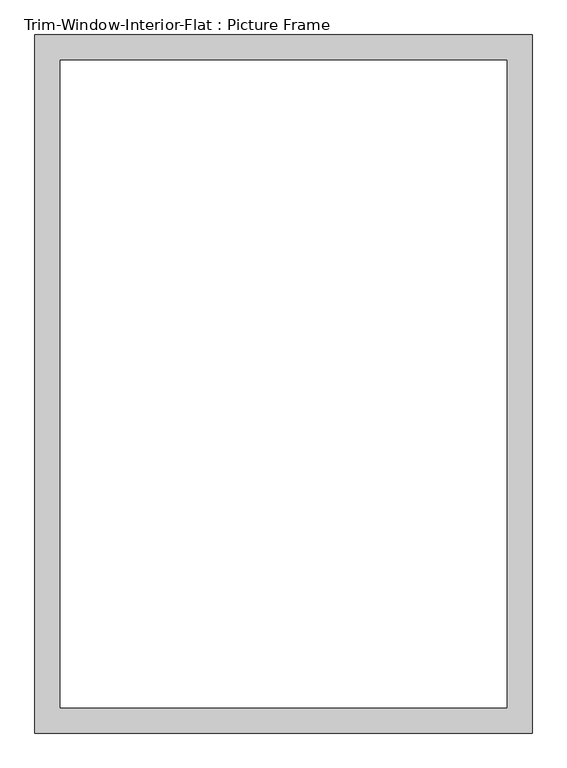
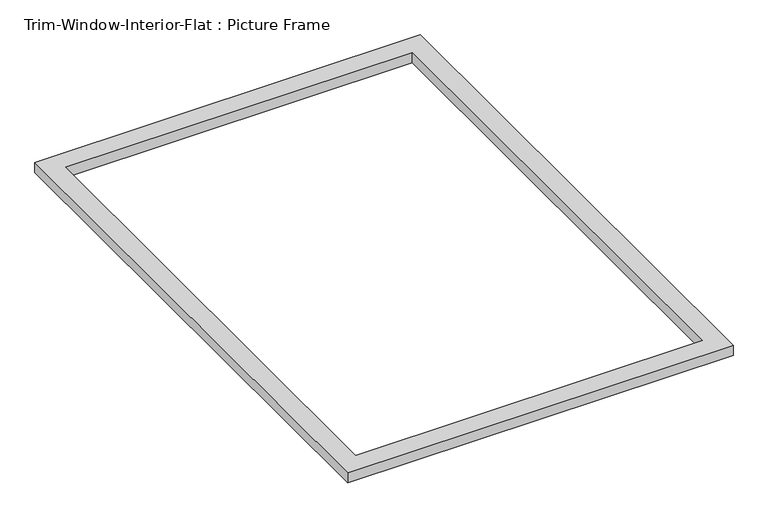
"""IFC4 building model written with IfcOpenShell, lengths in millimetres: proxy geometry, Trim-Window-Interior-Flat : Picture Frame."""

import ifcopenshell
import ifcopenshell.guid

model = None  # the IFC model being written
_history = None  # IfcOwnerHistory: only IFC2X3 demands one
_inside = {}  # id of a spatial element -> (the spatial element, [elements in it])
_under = {}  # id of a project, library or spatial element -> (it, [spatial elements below it])
_declared = {}  # id of a project -> (the project, [libraries it declares])
_typed = {}  # id of a type object -> (the type object, [elements of that type])
_made_of = {}  # id of a material, layer set ... -> (it, [elements and type objects made of it])


def new_model(schema):
    """Start an empty IFC model of exactly this schema.

    Asked for "IFC4X3", IfcOpenShell would pick the latest addendum, in which some entities
    have other attributes; the version numbers below select the first issue.
    IFC2X3 requires an IfcOwnerHistory on every rooted entity: one is made here for all.
    """
    global model, _history
    if schema == "IFC4X3":
        model = ifcopenshell.file(schema_version=(4, 3, 0, 0))
    else:
        model = ifcopenshell.file(schema=schema)
    _inside.clear()
    _under.clear()
    _declared.clear()
    _typed.clear()
    _made_of.clear()
    _history = None
    if model.schema == "IFC2X3":
        org = make("IfcOrganization", Name="unknown")
        user = make(
            "IfcPersonAndOrganization",
            ThePerson=make("IfcPerson", FamilyName="unknown"),
            TheOrganization=org,
        )
        app = make(
            "IfcApplication",
            ApplicationDeveloper=org,
            Version="unknown",
            ApplicationFullName="unknown",
            ApplicationIdentifier="unknown",
        )
        _history = make(
            "IfcOwnerHistory",
            OwningUser=user,
            OwningApplication=app,
            ChangeAction="ADDED",
            CreationDate=0,
        )
    return model


def make(cls, **values):
    """One entity of the class cls with the attributes given. An attribute that is None is left unset."""
    return model.create_entity(
        cls, **{name: value for name, value in values.items() if value is not None}
    )


def rooted(cls, **values):
    """An entity with a GlobalId (a new one), such as an element, a storey or a relation."""
    return make(cls, GlobalId=ifcopenshell.guid.new(), OwnerHistory=_history, **values)


def si_unit(unit_type, name, prefix=None):
    """IfcSIUnit, for example si_unit("LENGTHUNIT", "METRE", prefix="MILLI")."""
    return make("IfcSIUnit", UnitType=unit_type, Prefix=prefix, Name=name)


def assignment(units):
    """IfcUnitAssignment: the units of a project."""
    return None if units is None else make("IfcUnitAssignment", Units=units)


def point(xyz):
    """IfcCartesianPoint."""
    return None if xyz is None else make("IfcCartesianPoint", Coordinates=xyz)


def direction(xyz):
    """IfcDirection."""
    return None if xyz is None else make("IfcDirection", DirectionRatios=xyz)


def frame(location, z_axis=None, x_axis=None):
    """IfcAxis2Placement3D, a coordinate frame: its origin and axes. An axis left out is left unset."""
    return make(
        "IfcAxis2Placement3D",
        Location=point(location),
        Axis=direction(z_axis),
        RefDirection=direction(x_axis),
    )


def origin():
    """The frame at (0, 0, 0) with its axes left unset."""
    return frame((0.0, 0.0, 0.0))


def origin_with_axes():
    """The frame at (0, 0, 0) with the z axis (0, 0, 1) and the x axis (1, 0, 0) written out."""
    return frame((0.0, 0.0, 0.0), z_axis=(0.0, 0.0, 1.0), x_axis=(1.0, 0.0, 0.0))


def place(relative_to, where):
    """IfcLocalPlacement: puts the frame where relative to a parent placement (None: the world)."""
    return make(
        "IfcLocalPlacement", PlacementRelTo=relative_to, RelativePlacement=where
    )


def context(
    kind, dimensions, precision=None, world=None, true_north=None, identifier=None
):
    """IfcGeometricRepresentationContext, for example the 3D "Model" context."""
    return make(
        "IfcGeometricRepresentationContext",
        ContextIdentifier=identifier,
        ContextType=kind,
        CoordinateSpaceDimension=dimensions,
        Precision=precision,
        WorldCoordinateSystem=world,
        TrueNorth=true_north,
    )


def project(units=None, contexts=None):
    """IfcProject with its units and contexts."""
    return rooted(
        "IfcProject",
        Name="project",
        RepresentationContexts=contexts,
        UnitsInContext=assignment(units),
    )


def spatial(cls, under=None, at=None, **own):
    """A site, building, storey or space (cls), placed at a placement, below another one or the project."""
    s = rooted(cls, ObjectPlacement=at, **own)
    if under is not None:
        _under.setdefault(under.id(), (under, []))[1].append(s)
    return s


def polyline(points):
    """IfcPolyline through the points."""
    return make("IfcPolyline", Points=[point(p) for p in points])


def outline(outer, holes=None, kind="AREA"):
    """IfcArbitraryClosedProfileDef: a profile drawn as a closed curve; with holes, ...WithVoids."""
    if holes is None:
        return make("IfcArbitraryClosedProfileDef", ProfileType=kind, OuterCurve=outer)
    return make(
        "IfcArbitraryProfileDefWithVoids",
        ProfileType=kind,
        OuterCurve=outer,
        InnerCurves=holes,
    )


def extrude(swept, where, along, depth):
    """IfcExtrudedAreaSolid: the profile swept, set in the frame where, extruded along a direction by depth."""
    return make(
        "IfcExtrudedAreaSolid",
        SweptArea=swept,
        Position=where,
        ExtrudedDirection=direction(along),
        Depth=depth,
    )


def shape(context_of_items, identifier, shape_type, items):
    """IfcShapeRepresentation: the items that make up one representation, for example the "Body"."""
    return make(
        "IfcShapeRepresentation",
        ContextOfItems=context_of_items,
        RepresentationIdentifier=identifier,
        RepresentationType=shape_type,
        Items=items,
    )


def source(mapping_origin, context_of_items, identifier, shape_type, items):
    """IfcRepresentationMap: a shape defined once, which mapped items show again and again."""
    return make(
        "IfcRepresentationMap",
        MappingOrigin=mapping_origin,
        MappedRepresentation=shape(context_of_items, identifier, shape_type, items),
    )


def transform(
    local_origin,
    x_axis=None,
    y_axis=None,
    z_axis=None,
    scale=None,
    scale2=None,
    scale3=None,
    uniform=True,
):
    """IfcCartesianTransformationOperator3D, or its non-uniform kind. x_axis, y_axis, z_axis: its Axis1, 2, 3."""
    if uniform:
        return make(
            "IfcCartesianTransformationOperator3D",
            Axis1=direction(x_axis),
            Axis2=direction(y_axis),
            LocalOrigin=point(local_origin),
            Scale=scale,
            Axis3=direction(z_axis),
        )
    return make(
        "IfcCartesianTransformationOperator3DnonUniform",
        Axis1=direction(x_axis),
        Axis2=direction(y_axis),
        LocalOrigin=point(local_origin),
        Scale=scale,
        Axis3=direction(z_axis),
        Scale2=scale2,
        Scale3=scale3,
    )


def mapped(mapping_source, mapping_target):
    """IfcMappedItem: shows the shape of a source again, moved by a transform."""
    return make(
        "IfcMappedItem", MappingSource=mapping_source, MappingTarget=mapping_target
    )


def made_of(thing, what):
    """Note that an element or type object is made of a material, layer set ...; save() writes the relation."""
    if what is not None:
        _made_of.setdefault(what.id(), (what, []))[1].append(thing)
    return thing


def element(
    cls,
    number,
    at=None,
    inside=None,
    cuts=None,
    type_object=None,
    material=None,
    context=None,
    identifier="Body",
    shape_type=None,
    held_by="IfcProductDefinitionShape",
    body=None,
    shapes=None,
    **own,
):
    """One element of the class cls, such as IfcWall. Its Tag is "e" and its number.

    at: its placement. inside: the storey or other place that contains it. cuts: it is an
    opening in that element (IfcRelVoidsElement). A single representation is given by context,
    identifier, shape_type and body (its items); several are given by shapes. held_by: the class
    of the entity that holds the representations. save() writes the other relations.
    """
    e = rooted(cls, Tag="e%d" % number, ObjectPlacement=at, **own)
    if body is not None:
        shapes = [shape(context, identifier, shape_type, body)]
    if shapes is not None:
        e.Representation = make(held_by, Representations=shapes)
    if inside is not None:
        _inside.setdefault(inside.id(), (inside, []))[1].append(e)
    if cuts is not None:
        rooted(
            "IfcRelVoidsElement", RelatingBuildingElement=cuts, RelatedOpeningElement=e
        )
    if type_object is not None:
        _typed.setdefault(type_object.id(), (type_object, []))[1].append(e)
    return made_of(e, material)


def aggregate(whole, parts):
    """IfcRelAggregates: a whole, such as a stair, and the parts it consists of."""
    return rooted("IfcRelAggregates", RelatingObject=whole, RelatedObjects=parts)


def save(model, path):
    """Write the relations noted so far, then the file.

    IfcRelAggregates (storeys below a building ...), IfcRelContainedInSpatialStructure (elements
    in a storey), IfcRelDefinesByType, IfcRelAssociatesMaterial and IfcRelDeclares: one each for
    every whole, place, type object, material and project.
    """
    for whole, parts in _under.values():
        aggregate(whole, parts)
    for where, things in _inside.values():
        rooted(
            "IfcRelContainedInSpatialStructure",
            RelatedElements=things,
            RelatingStructure=where,
        )
    for kind, things in _typed.values():
        rooted("IfcRelDefinesByType", RelatedObjects=things, RelatingType=kind)
    for what, things in _made_of.values():
        rooted("IfcRelAssociatesMaterial", RelatedObjects=things, RelatingMaterial=what)
    for by, libraries in _declared.values():
        rooted("IfcRelDeclares", RelatingContext=by, RelatedDefinitions=libraries)
    model.write(path)


def trim_window_interior_flat_picture_frame_208726ef(model_context):
    return source(origin(), model_context, "Body", "SweptSolid", [
        extrude(outline(polyline([(565.15, 44.45), (565.15, -1543.05), (-565.15, -1543.05), (-565.15, 44.45), (565.15, 44.45)]), holes=[polyline([(508.0, -12.7), (-508.0, -12.7), (-508.0, -1485.9), (508.0, -1485.9), (508.0, -12.7)])]), origin_with_axes(), (0.0, 0.0, 1.0), 31.75),
    ])


if __name__ == "__main__":
    model = new_model("IFC4")
    model_context = context("Model", 3, world=origin())
    ifc_project = project(units=[si_unit("LENGTHUNIT", "METRE", prefix="MILLI")], contexts=[model_context])
    site = spatial("IfcSite", under=ifc_project)
    building = spatial("IfcBuilding", under=site)
    placement = place(None, origin())
    trim_window_interior_flat_picture_frame_shape = trim_window_interior_flat_picture_frame_208726ef(model_context)
    element("IfcBuildingElementProxy", 1, Name="Trim-Window-Interior-Flat : Picture Frame", ObjectType="Trim-Window-Interior-Flat : Picture Frame", at=placement, inside=building, context=model_context, shape_type="MappedRepresentation", body=[
        mapped(trim_window_interior_flat_picture_frame_shape, transform((0.0, 0.0, 0.0), x_axis=(1.0, 0.0, 0.0), y_axis=(0.0, 1.0, 0.0), z_axis=(0.0, 0.0, 1.0))),
    ])
    save(model, "model.ifc")

# Revit data of these elements
# Type "Trim-Window-Interior-Flat : Picture Frame"
#   Trim Thickness_Picture Frame = 0' - 1 1/4"
#   Trim Width = 0' - 2 1/4"
#   Trim Thickness_with Sill = 0' - 0 3/4"
#   Sill Thickness = 0' - 1 1/4"
#   Opening Width [instance default] = 2' - 0"
#   Opening Height [instance default] = 3' - 0"
#   Default Elevation = 4' - 0"
#   Sill = no
#   Picture Frame = yes
#   Trim Material [instance default] = none
# Element 1 (IfcBuildingElementProxy, "Trim-Window-Interior-Flat : Picture Frame")
#   Opening Width = 3' - 5"
#   Opening Height = 4' - 11"
#   Trim Material = Wood - Stained
#   Materials on its faces: "Wood - Stained"
# Materials
#   "Wood - Stained": class "Wood", colour RGB 224 178 126, transparency 0, Cost = 0
